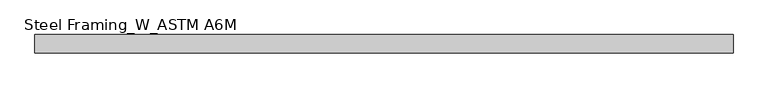
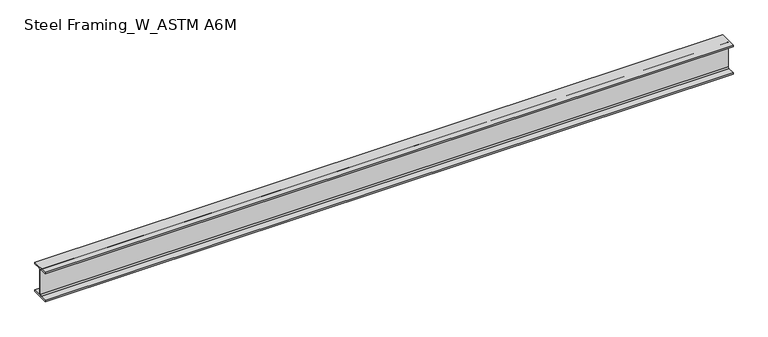
"""IFC4 building model written with IfcOpenShell, lengths in millimetres: beam geometry, Steel Framing_W_ASTM A6M : H_SB_AR_S02_W360x79_RB2A."""

from ifc_helpers import new_model, si_unit, point, frame, frame_2d, origin, place, context, project, spatial, polyline, circle_curve, trimmed, segment, composite_curve, outline, extrude, source, transform, mapped, element, save


def steel_framing_w_astm_a6m_13680513(model_context):
    return source(origin(), model_context, "Body", "SweptSolid", [
        extrude(outline(composite_curve([segment(polyline([(102.5, -159.7), (102.5, -176.5), (-102.5, -176.5), (-102.5, -159.7), (-19.7, -159.7)]), True, "CONTINUOUS"), segment(trimmed(circle_curve(frame_2d((-19.7, -144.7)), 15.0), [point((-19.7, -159.7))], [point((-4.7, -144.7))], True, "CARTESIAN"), True, "CONTINUOUS"), segment(polyline([(-4.7, -144.7), (-4.7, 144.7)]), True, "CONTINUOUS"), segment(trimmed(circle_curve(frame_2d((-19.7, 144.7)), 15.0), [point((-4.7, 144.7))], [point((-19.7, 159.7))], True, "CARTESIAN"), True, "CONTINUOUS"), segment(polyline([(-19.7, 159.7), (-102.5, 159.7), (-102.5, 176.5), (102.5, 176.5), (102.5, 159.7), (19.7, 159.7)]), True, "CONTINUOUS"), segment(trimmed(circle_curve(frame_2d((19.7, 144.7)), 15.0), [point((19.7, 159.7))], [point((4.7, 144.7))], True, "CARTESIAN"), True, "CONTINUOUS"), segment(polyline([(4.7, 144.7), (4.7, -144.7)]), True, "CONTINUOUS"), segment(trimmed(circle_curve(frame_2d((19.7, -144.7)), 15.0), [point((4.7, -144.7))], [point((19.7, -159.7))], True, "CARTESIAN"), True, "CONTINUOUS"), segment(polyline([(19.7, -159.7), (102.5, -159.7)]), True, "CONTINUOUS")], self_intersect=False)), frame((-3866.4, 0.0, 0.0), z_axis=(1.0, 0.0, 0.0), x_axis=(0.0, 1.0, 0.0)), (0.0, 0.0, 1.0), 7873.6),
    ])


if __name__ == "__main__":
    model = new_model("IFC4")
    model_context = context("Model", 3, world=origin())
    ifc_project = project(units=[si_unit("LENGTHUNIT", "METRE", prefix="MILLI")], contexts=[model_context])
    site = spatial("IfcSite", under=ifc_project)
    building = spatial("IfcBuilding", under=site)
    placement = place(None, origin())
    steel_framing_w_astm_a6m_shape = steel_framing_w_astm_a6m_13680513(model_context)
    element("IfcBeam", 1, ObjectType="Steel Framing_W_ASTM A6M : H_SB_AR_S02_W360x79_RB2A", at=placement, inside=building, context=model_context, shape_type="MappedRepresentation", body=[
        mapped(steel_framing_w_astm_a6m_shape, transform((0.0, 0.0, 0.0), x_axis=(1.0, 0.0, 0.0), y_axis=(0.0, 1.0, 0.0), z_axis=(0.0, 0.0, 1.0))),
    ])
    save(model, "model.ifc")

# Revit data of these elements
# Type "Steel Framing_W_ASTM A6M : H_SB_AR_S02_W360x79_RB2A"
#   Type Mark = "RB2A"
#   Section Name Key = "W14x53"
#   Width = 20.5 cm
#   Web Thickness = 0.94 cm
#   Web Fillet = 1.5 cm
#   Warping Constant = 682000.0 cm⁶
#   Torsional Moment of Inertia = 80.70 cm⁴
#   Section Area = 101.0 cm²
#   Plastic Modulus weak axis = 361.0 cm³
#   Plastic Modulus strong axis = 1430.0 cm³
#   Perimeter = 1.48 m²/m
#   Nominal Weight = 79.00 kgf/m
#   Moment of Inertia weak axis = 2400.00 cm⁴
#   Moment of Inertia strong axis = 22500.00 cm⁴
#   Height = 35.3 cm
#   Flange Thickness = 1.68 cm
#   Elastic Modulus weak axis = 234.0 cm³
#   Elastic Modulus strong axis = 1270.0 cm³
#   Centroid Vertical = 17.65 cm
#   Centroid Horizontal = 10.25 cm
#   Length [instance default] = 1500 mm
#   Structural Material [instance default] = Steel, 45-345
#   Bolt Spacing = 0
#   Assembly Code = ""
# Element 1 (IfcBeam, "Steel Framing_W_ASTM A6M : H_SB_AR_S02_W360x79_RB2A")
#   Materials on its faces: "Steel, 45-345"
# Materials
#   "Steel, 45-345": class "Metal", colour RGB 189 187 185, transparency 0, Description = "Steel 345 MPa", Cost = 0
